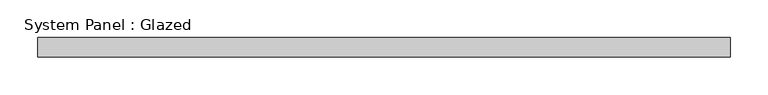
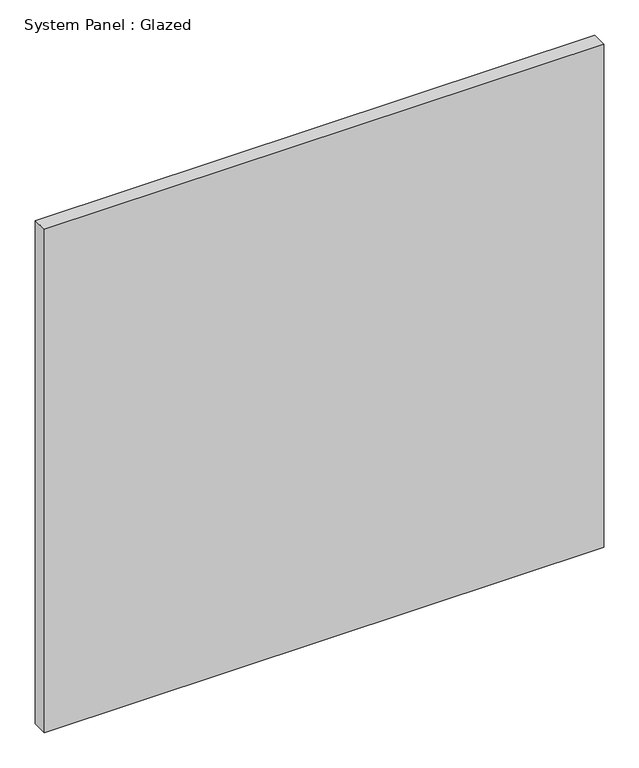
"""IFC4 building model written with IfcOpenShell, lengths in millimetres: plate geometry, System Panel : Glazed."""

from ifc_helpers import new_model, si_unit, origin, origin_with_axes, place, context, project, spatial, polyline, outline, extrude, source, transform, mapped, element, save


def system_panel_glazed_652e8fc4(model_context):
    return source(origin(), model_context, "Body", "SweptSolid", [
        extrude(outline(polyline([(457.2, -44.45), (-457.2, -44.45), (-457.2, -19.05), (457.2, -19.05), (457.2, -44.45)])), origin_with_axes(), (0.0, 0.0, 1.0), 869.95),
    ])


if __name__ == "__main__":
    model = new_model("IFC4")
    model_context = context("Model", 3, world=origin())
    ifc_project = project(units=[si_unit("LENGTHUNIT", "METRE", prefix="MILLI")], contexts=[model_context])
    site = spatial("IfcSite", under=ifc_project)
    building = spatial("IfcBuilding", under=site)
    placement = place(None, origin())
    system_panel_glazed_shape = system_panel_glazed_652e8fc4(model_context)
    element("IfcPlate", 1, ObjectType="System Panel : Glazed", at=placement, inside=building, context=model_context, shape_type="MappedRepresentation", body=[
        mapped(system_panel_glazed_shape, transform((0.0, 0.0, 0.0), x_axis=(1.0, 0.0, 0.0), y_axis=(0.0, 1.0, 0.0), z_axis=(0.0, 0.0, 1.0))),
    ])
    save(model, "model.ifc")

# Revit data of these elements
# Element 1 (IfcPlate, "System Panel : Glazed")
#   Materials on its faces: "Glass"
# Materials
#   "Glass": class "Glass", colour RGB 0 128 192, transparency 0.75
